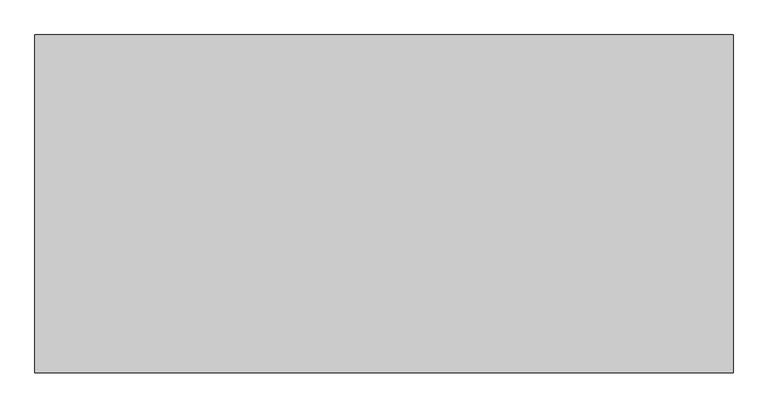
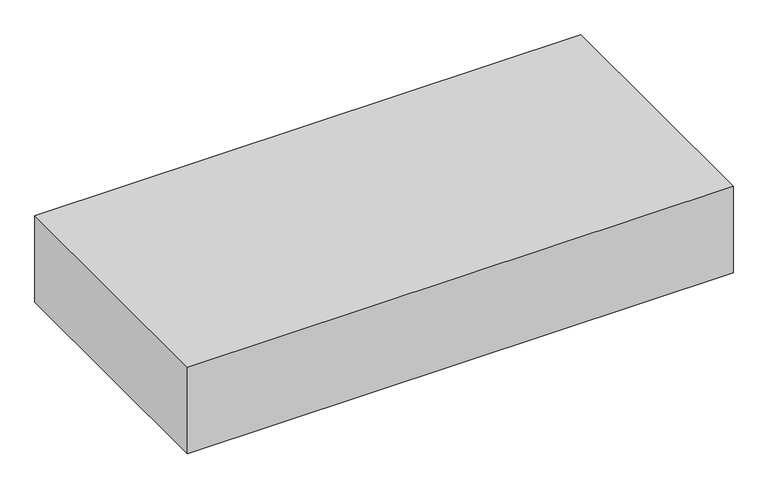
"""IFC4 building model written with IfcOpenShell, lengths in millimetres: proxy geometry, Space Planning Box_hec : Space Planning Box_hec."""

import ifcopenshell
import ifcopenshell.guid

model = None  # the IFC model being written
_history = None  # IfcOwnerHistory: only IFC2X3 demands one
_inside = {}  # id of a spatial element -> (the spatial element, [elements in it])
_under = {}  # id of a project, library or spatial element -> (it, [spatial elements below it])
_declared = {}  # id of a project -> (the project, [libraries it declares])
_typed = {}  # id of a type object -> (the type object, [elements of that type])
_made_of = {}  # id of a material, layer set ... -> (it, [elements and type objects made of it])


def new_model(schema):
    """Start an empty IFC model of exactly this schema.

    Asked for "IFC4X3", IfcOpenShell would pick the latest addendum, in which some entities
    have other attributes; the version numbers below select the first issue.
    IFC2X3 requires an IfcOwnerHistory on every rooted entity: one is made here for all.
    """
    global model, _history
    if schema == "IFC4X3":
        model = ifcopenshell.file(schema_version=(4, 3, 0, 0))
    else:
        model = ifcopenshell.file(schema=schema)
    _inside.clear()
    _under.clear()
    _declared.clear()
    _typed.clear()
    _made_of.clear()
    _history = None
    if model.schema == "IFC2X3":
        org = make("IfcOrganization", Name="unknown")
        user = make(
            "IfcPersonAndOrganization",
            ThePerson=make("IfcPerson", FamilyName="unknown"),
            TheOrganization=org,
        )
        app = make(
            "IfcApplication",
            ApplicationDeveloper=org,
            Version="unknown",
            ApplicationFullName="unknown",
            ApplicationIdentifier="unknown",
        )
        _history = make(
            "IfcOwnerHistory",
            OwningUser=user,
            OwningApplication=app,
            ChangeAction="ADDED",
            CreationDate=0,
        )
    return model


def make(cls, **values):
    """One entity of the class cls with the attributes given. An attribute that is None is left unset."""
    return model.create_entity(
        cls, **{name: value for name, value in values.items() if value is not None}
    )


def rooted(cls, **values):
    """An entity with a GlobalId (a new one), such as an element, a storey or a relation."""
    return make(cls, GlobalId=ifcopenshell.guid.new(), OwnerHistory=_history, **values)


def si_unit(unit_type, name, prefix=None):
    """IfcSIUnit, for example si_unit("LENGTHUNIT", "METRE", prefix="MILLI")."""
    return make("IfcSIUnit", UnitType=unit_type, Prefix=prefix, Name=name)


def assignment(units):
    """IfcUnitAssignment: the units of a project."""
    return None if units is None else make("IfcUnitAssignment", Units=units)


def point(xyz):
    """IfcCartesianPoint."""
    return None if xyz is None else make("IfcCartesianPoint", Coordinates=xyz)


def direction(xyz):
    """IfcDirection."""
    return None if xyz is None else make("IfcDirection", DirectionRatios=xyz)


def frame(location, z_axis=None, x_axis=None):
    """IfcAxis2Placement3D, a coordinate frame: its origin and axes. An axis left out is left unset."""
    return make(
        "IfcAxis2Placement3D",
        Location=point(location),
        Axis=direction(z_axis),
        RefDirection=direction(x_axis),
    )


def origin():
    """The frame at (0, 0, 0) with its axes left unset."""
    return frame((0.0, 0.0, 0.0))


def origin_with_axes():
    """The frame at (0, 0, 0) with the z axis (0, 0, 1) and the x axis (1, 0, 0) written out."""
    return frame((0.0, 0.0, 0.0), z_axis=(0.0, 0.0, 1.0), x_axis=(1.0, 0.0, 0.0))


def place(relative_to, where):
    """IfcLocalPlacement: puts the frame where relative to a parent placement (None: the world)."""
    return make(
        "IfcLocalPlacement", PlacementRelTo=relative_to, RelativePlacement=where
    )


def context(
    kind, dimensions, precision=None, world=None, true_north=None, identifier=None
):
    """IfcGeometricRepresentationContext, for example the 3D "Model" context."""
    return make(
        "IfcGeometricRepresentationContext",
        ContextIdentifier=identifier,
        ContextType=kind,
        CoordinateSpaceDimension=dimensions,
        Precision=precision,
        WorldCoordinateSystem=world,
        TrueNorth=true_north,
    )


def project(units=None, contexts=None):
    """IfcProject with its units and contexts."""
    return rooted(
        "IfcProject",
        Name="project",
        RepresentationContexts=contexts,
        UnitsInContext=assignment(units),
    )


def spatial(cls, under=None, at=None, **own):
    """A site, building, storey or space (cls), placed at a placement, below another one or the project."""
    s = rooted(cls, ObjectPlacement=at, **own)
    if under is not None:
        _under.setdefault(under.id(), (under, []))[1].append(s)
    return s


def polyline(points):
    """IfcPolyline through the points."""
    return make("IfcPolyline", Points=[point(p) for p in points])


def outline(outer, holes=None, kind="AREA"):
    """IfcArbitraryClosedProfileDef: a profile drawn as a closed curve; with holes, ...WithVoids."""
    if holes is None:
        return make("IfcArbitraryClosedProfileDef", ProfileType=kind, OuterCurve=outer)
    return make(
        "IfcArbitraryProfileDefWithVoids",
        ProfileType=kind,
        OuterCurve=outer,
        InnerCurves=holes,
    )


def extrude(swept, where, along, depth):
    """IfcExtrudedAreaSolid: the profile swept, set in the frame where, extruded along a direction by depth."""
    return make(
        "IfcExtrudedAreaSolid",
        SweptArea=swept,
        Position=where,
        ExtrudedDirection=direction(along),
        Depth=depth,
    )


def shape(context_of_items, identifier, shape_type, items):
    """IfcShapeRepresentation: the items that make up one representation, for example the "Body"."""
    return make(
        "IfcShapeRepresentation",
        ContextOfItems=context_of_items,
        RepresentationIdentifier=identifier,
        RepresentationType=shape_type,
        Items=items,
    )


def source(mapping_origin, context_of_items, identifier, shape_type, items):
    """IfcRepresentationMap: a shape defined once, which mapped items show again and again."""
    return make(
        "IfcRepresentationMap",
        MappingOrigin=mapping_origin,
        MappedRepresentation=shape(context_of_items, identifier, shape_type, items),
    )


def transform(
    local_origin,
    x_axis=None,
    y_axis=None,
    z_axis=None,
    scale=None,
    scale2=None,
    scale3=None,
    uniform=True,
):
    """IfcCartesianTransformationOperator3D, or its non-uniform kind. x_axis, y_axis, z_axis: its Axis1, 2, 3."""
    if uniform:
        return make(
            "IfcCartesianTransformationOperator3D",
            Axis1=direction(x_axis),
            Axis2=direction(y_axis),
            LocalOrigin=point(local_origin),
            Scale=scale,
            Axis3=direction(z_axis),
        )
    return make(
        "IfcCartesianTransformationOperator3DnonUniform",
        Axis1=direction(x_axis),
        Axis2=direction(y_axis),
        LocalOrigin=point(local_origin),
        Scale=scale,
        Axis3=direction(z_axis),
        Scale2=scale2,
        Scale3=scale3,
    )


def mapped(mapping_source, mapping_target):
    """IfcMappedItem: shows the shape of a source again, moved by a transform."""
    return make(
        "IfcMappedItem", MappingSource=mapping_source, MappingTarget=mapping_target
    )


def made_of(thing, what):
    """Note that an element or type object is made of a material, layer set ...; save() writes the relation."""
    if what is not None:
        _made_of.setdefault(what.id(), (what, []))[1].append(thing)
    return thing


def element(
    cls,
    number,
    at=None,
    inside=None,
    cuts=None,
    type_object=None,
    material=None,
    context=None,
    identifier="Body",
    shape_type=None,
    held_by="IfcProductDefinitionShape",
    body=None,
    shapes=None,
    **own,
):
    """One element of the class cls, such as IfcWall. Its Tag is "e" and its number.

    at: its placement. inside: the storey or other place that contains it. cuts: it is an
    opening in that element (IfcRelVoidsElement). A single representation is given by context,
    identifier, shape_type and body (its items); several are given by shapes. held_by: the class
    of the entity that holds the representations. save() writes the other relations.
    """
    e = rooted(cls, Tag="e%d" % number, ObjectPlacement=at, **own)
    if body is not None:
        shapes = [shape(context, identifier, shape_type, body)]
    if shapes is not None:
        e.Representation = make(held_by, Representations=shapes)
    if inside is not None:
        _inside.setdefault(inside.id(), (inside, []))[1].append(e)
    if cuts is not None:
        rooted(
            "IfcRelVoidsElement", RelatingBuildingElement=cuts, RelatedOpeningElement=e
        )
    if type_object is not None:
        _typed.setdefault(type_object.id(), (type_object, []))[1].append(e)
    return made_of(e, material)


def aggregate(whole, parts):
    """IfcRelAggregates: a whole, such as a stair, and the parts it consists of."""
    return rooted("IfcRelAggregates", RelatingObject=whole, RelatedObjects=parts)


def save(model, path):
    """Write the relations noted so far, then the file.

    IfcRelAggregates (storeys below a building ...), IfcRelContainedInSpatialStructure (elements
    in a storey), IfcRelDefinesByType, IfcRelAssociatesMaterial and IfcRelDeclares: one each for
    every whole, place, type object, material and project.
    """
    for whole, parts in _under.values():
        aggregate(whole, parts)
    for where, things in _inside.values():
        rooted(
            "IfcRelContainedInSpatialStructure",
            RelatedElements=things,
            RelatingStructure=where,
        )
    for kind, things in _typed.values():
        rooted("IfcRelDefinesByType", RelatedObjects=things, RelatingType=kind)
    for what, things in _made_of.values():
        rooted("IfcRelAssociatesMaterial", RelatedObjects=things, RelatingMaterial=what)
    for by, libraries in _declared.values():
        rooted("IfcRelDeclares", RelatingContext=by, RelatedDefinitions=libraries)
    model.write(path)


def generic_models_32ca781f(model_context):
    return source(origin(), model_context, "Body", "SweptSolid", [
        extrude(outline(polyline([(15500.0, 7500.0), (15500.0, -7500.0), (-15500.0, -7500.0), (-15500.0, 7500.0), (15500.0, 7500.0)])), origin_with_axes(), (0.0, 0.0, 1.0), 5200.0),
    ])


if __name__ == "__main__":
    model = new_model("IFC4")
    model_context = context("Model", 3, world=origin())
    ifc_project = project(units=[si_unit("LENGTHUNIT", "METRE", prefix="MILLI")], contexts=[model_context])
    site = spatial("IfcSite", under=ifc_project)
    building = spatial("IfcBuilding", under=site)
    placement = place(None, origin())
    generic_models_shape = generic_models_32ca781f(model_context)
    element("IfcBuildingElementProxy", 1, Name="Space Planning Box_hec : Space Planning Box_hec", ObjectType="Space Planning Box_hec : Space Planning Box_hec", at=placement, inside=building, context=model_context, shape_type="MappedRepresentation", body=[
        mapped(generic_models_shape, transform((0.0, 0.0, 0.0), x_axis=(1.0, 0.0, 0.0), y_axis=(0.0, 1.0, 0.0), z_axis=(0.0, 0.0, 1.0))),
    ])
    save(model, "model.ifc")

# Revit data of these elements
# Type "Space Planning Box_hec : Space Planning Box_hec"
#   Type Comments = "..."
#   Room Name [instance default] = "?"
#   Interior Finish [instance default] = ""
#   Exterior Finish [instance default] = ""
#   Department [instance default] = ""
#   Assembly Code = "..."
#   ceiling height [instance default] = 0
#   Width [instance default] = 1524 mm
#   Program Area [instance default] = 0.00 m²
#   Length [instance default] = 1524 mm
#   Height [instance default] = 1524 mm
#   Area [instance default] = 2.32258 m²
#   Fill Color [instance default] = Cyan
#   Default Elevation = 0
# Element 1 (IfcBuildingElementProxy, "Space Planning Box_hec : Space Planning Box_hec")
#   Room Name = "Electrical Room"
#   Interior Finish = "IW1..N/A,,WB1..N/A,,FL2..N/A,,CL1..N/A"
#   Exterior Finish = "N/A..N/A,,EW1..N/A"
#   Department = "EL"
#   Width = 31000 mm
#   Program Area = 465.00 m²
#   Length = 15000 mm
#   Height = 5200 mm
#   Area = 465.00 m²
#   Fill Color = Orange
#   Materials on its faces: "Orange"
# Materials
#   "Cyan": class "Generic", colour RGB 0 255 255, transparency 0.2, Cost = 0
#   "Orange": class "Generic", colour RGB 255 165 0, transparency 0.2, Cost = 0
